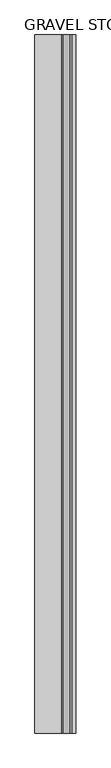
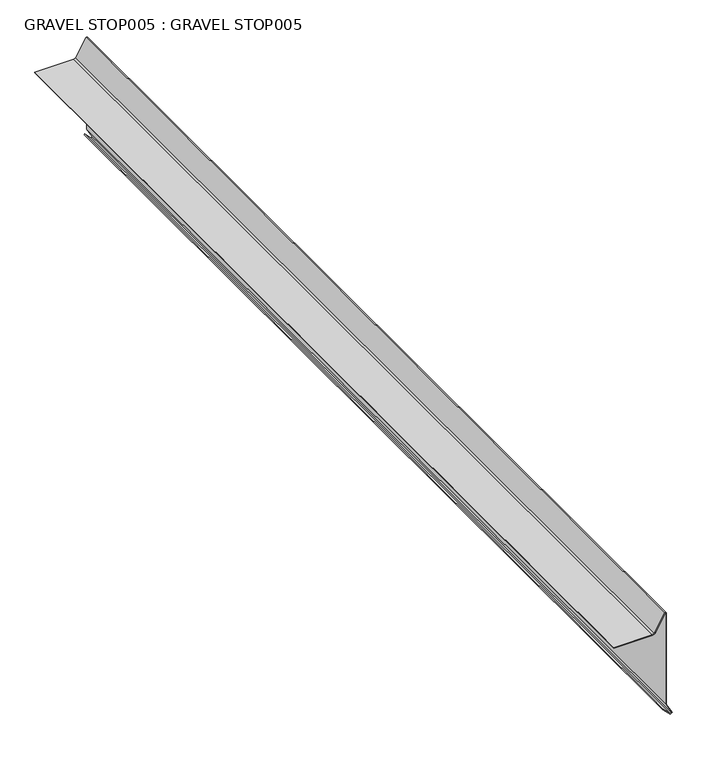
"""IFC4 building model written with IfcOpenShell, lengths in millimetres: proxy geometry, GRAVEL STOP005 : GRAVEL STOP005."""

from ifc_helpers import new_model, si_unit, frame, origin, place, context, project, spatial, polyline, outline, extrude, source, transform, mapped, element, save


def gravel_stop005_gravel_stop005_bb7cdfd3(model_context):
    return source(origin(), model_context, "Body", "SweptSolid", [
        extrude(outline(polyline([(40077.410403, -4353.4420496), (40080.5182783, -4349.3681054), (40101.8558531, -4361.0170744), (40294.5307525, -4361.0170744), (40295.3431515, -4364.0489887), (40259.5408757, -4384.7194423), (40257.3744784, -4388.4717525), (40257.3744784, -4465.9296592), (40255.9633674, -4465.9296592), (40255.9633674, -4388.0936464), (40258.5078708, -4383.6864373), (40293.699878, -4363.3683225), (40293.447969, -4362.4281854), (40101.495749, -4362.4281854), (40080.9054201, -4351.1871656), (40079.2807815, -4353.3168157), (40092.8027062, -4366.8387404), (40091.8049, -4367.8365465), (40077.410403, -4353.4420496)])), frame((0.0, -1065.5906573, 0.0), z_axis=(0.0, 1.0, 0.0), x_axis=(0.0, 0.0, 1.0)), (0.0, 0.0, 1.0), 2000.25),
    ])


if __name__ == "__main__":
    model = new_model("IFC4")
    model_context = context("Model", 3, world=origin())
    ifc_project = project(units=[si_unit("LENGTHUNIT", "METRE", prefix="MILLI")], contexts=[model_context])
    site = spatial("IfcSite", under=ifc_project)
    building = spatial("IfcBuilding", under=site)
    placement = place(None, origin())
    gravel_stop005_gravel_stop005_shape = gravel_stop005_gravel_stop005_bb7cdfd3(model_context)
    element("IfcBuildingElementProxy", 1, Name="GRAVEL STOP005 : GRAVEL STOP005", ObjectType="GRAVEL STOP005 : GRAVEL STOP005", at=placement, inside=building, context=model_context, shape_type="MappedRepresentation", body=[
        mapped(gravel_stop005_gravel_stop005_shape, transform((0.0, 0.0, 0.0), x_axis=(1.0, 0.0, 0.0), y_axis=(0.0, 1.0, 0.0), z_axis=(0.0, 0.0, 1.0))),
    ])
    save(model, "model.ifc")

# Revit data of these elements
# Type "GRAVEL STOP005 : GRAVEL STOP005"
#   NameOverride = "GRAVEL STOP005"
# Element 1 (IfcBuildingElementProxy, "GRAVEL STOP005 : GRAVEL STOP005")
#   Materials on its faces: "GRAVEL STOP REQUIRED WITH GRAVEL SURFACE SYSTEMS"
# Materials
#   "GRAVEL STOP REQUIRED WITH GRAVEL SURFACE SYSTEMS": class "Unassigned", colour RGB 170 170 127, transparency 0
